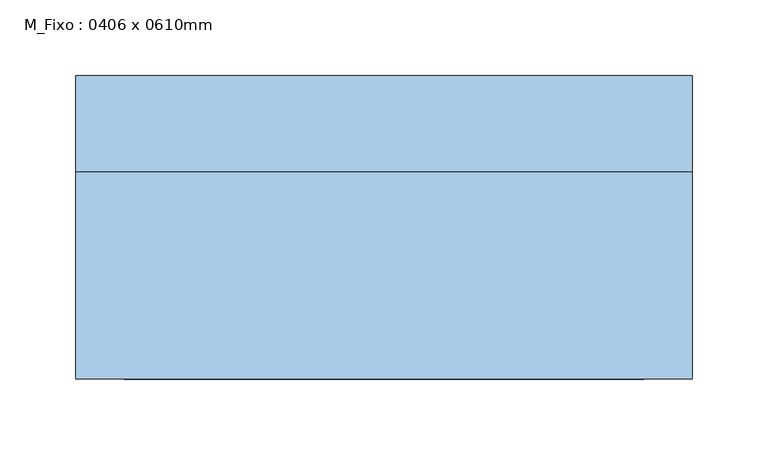
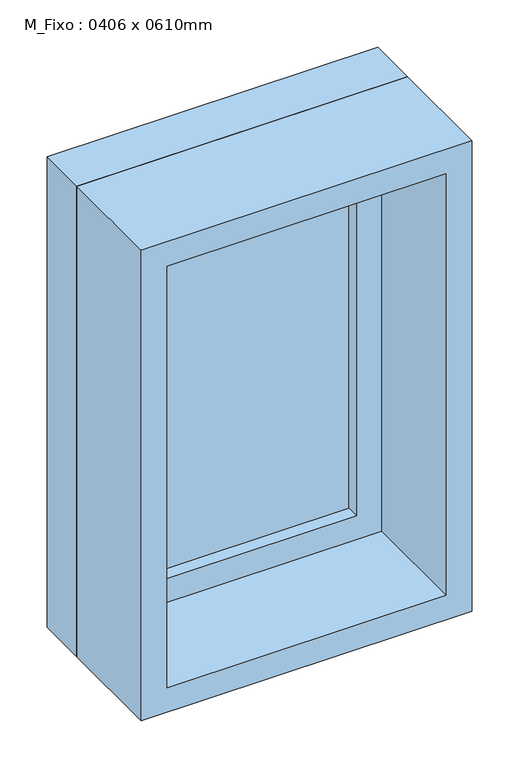
"""IFC4 building model written with IfcOpenShell, lengths in millimetres: window geometry, M_Fixo : 0406 x 0610mm."""

from ifc_helpers import new_model, si_unit, frame, origin, place, context, project, spatial, polyline, outline, extrude, source, transform, mapped, element, save


def m_fixo_0406_x_0610mm_8205b201(model_context):
    return source(origin(), model_context, "Body", "SweptSolid", [
        extrude(outline(polyline([(-140.0, 78.0), (140.0, 78.0), (140.0, 66.0), (-140.0, 66.0), (-140.0, 78.0)])), frame((0.0, 0.0, 978.0), z_axis=(0.0, 0.0, 1.0), x_axis=(1.0, 0.0, 0.0)), (0.0, 0.0, 1.0), 484.0),
        extrude(outline(polyline([(1506.0, -184.0), (934.0, -184.0), (934.0, 184.0), (1506.0, 184.0), (1506.0, -184.0)]), holes=[polyline([(1462.0, -140.0), (1462.0, 140.0), (978.0, 140.0), (978.0, -140.0), (1462.0, -140.0)])]), frame((0.0, 50.0, 0.0), z_axis=(0.0, 1.0, 0.0), x_axis=(0.0, 0.0, 1.0)), (0.0, 0.0, 1.0), 44.0),
        extrude(outline(polyline([(1525.0, -203.0), (915.0, -203.0), (915.0, 203.0), (1525.0, 203.0), (1525.0, -203.0)]), holes=[polyline([(1506.0, -184.0), (1506.0, 184.0), (934.0, 184.0), (934.0, -184.0), (1506.0, -184.0)])]), frame((0.0, 50.0, 0.0), z_axis=(0.0, 1.0, 0.0), x_axis=(0.0, 0.0, 1.0)), (0.0, 0.0, 1.0), 63.0),
        extrude(outline(polyline([(1525.0, -203.0), (915.0, -203.0), (915.0, 203.0), (1525.0, 203.0), (1525.0, -203.0)]), holes=[polyline([(1493.0, -171.0), (1493.0, 171.0), (947.0, 171.0), (947.0, -171.0), (1493.0, -171.0)])]), frame((0.0, -87.0, 0.0), z_axis=(0.0, 1.0, 0.0), x_axis=(0.0, 0.0, 1.0)), (0.0, 0.0, 1.0), 137.0),
    ])


if __name__ == "__main__":
    model = new_model("IFC4")
    model_context = context("Model", 3, world=origin())
    ifc_project = project(units=[si_unit("LENGTHUNIT", "METRE", prefix="MILLI")], contexts=[model_context])
    site = spatial("IfcSite", under=ifc_project)
    building = spatial("IfcBuilding", under=site)
    placement = place(None, origin())
    m_fixo_0406_x_0610mm_shape = m_fixo_0406_x_0610mm_8205b201(model_context)
    element("IfcWindow", 1, ObjectType="M_Fixo : 0406 x 0610mm", at=placement, inside=building, context=model_context, shape_type="MappedRepresentation", body=[
        mapped(m_fixo_0406_x_0610mm_shape, transform((0.0, 0.0, 0.0), x_axis=(1.0, 0.0, 0.0), y_axis=(0.0, 1.0, 0.0), z_axis=(0.0, 0.0, 1.0))),
    ])
    save(model, "model.ifc")

# Revit data of these elements
# Type "M_Fixo : 0406 x 0610mm"
#   Type Mark = "10"
#   Construction Type Id = "GSP4R"
#   Analytic Construction = "Vidraça única Pilkington 1/8 pol"
#   Visual Light Transmittance = 0.9
#   Thermal Resistance (R) = 0.271106 (m²·K)/W
#   Solar Heat Gain Coefficient = 0.78
#   Heat Transfer Coefficient (U) = 3.6886 W/(m²·K)
#   Height = 0.61 m
#   Altura-padrão do peitoril = 0.915 m
#   Width = 0.406 m
#   Janela aplicada = 0.019 m
#   Define Thermal Properties by = 1
#   Material da estrutura externa = Caixilho
#   Material da estrutura interna = Caixilho
#   Material do painel de vidro = Vidro
#   Caixilho = Caixilho
#   Wall Closure = (empty or 0)
# Element 1 (IfcWindow, "M_Fixo : 0406 x 0610mm")
#   Materials on its faces: "Caixilho", "Vidro"
# Materials
#   "Caixilho": class "Madeira", colour RGB 224 178 126, transparency 0, Cost = 0
#   "Vidro": class "Vidro", colour RGB 0 128 192, transparency 0.9, Description = "Vidro de sílica", Cost = 0
